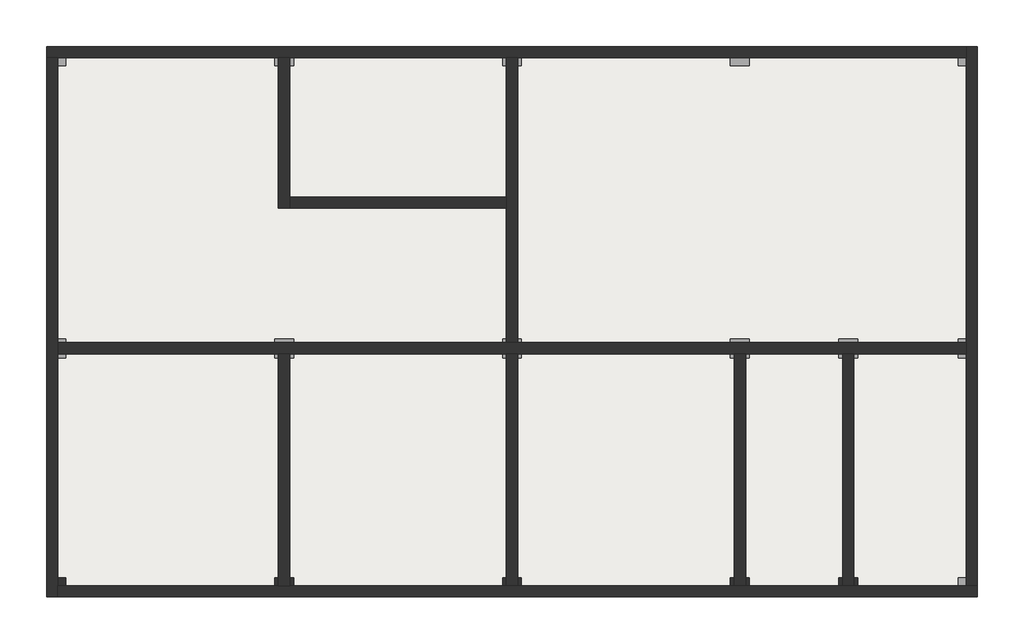
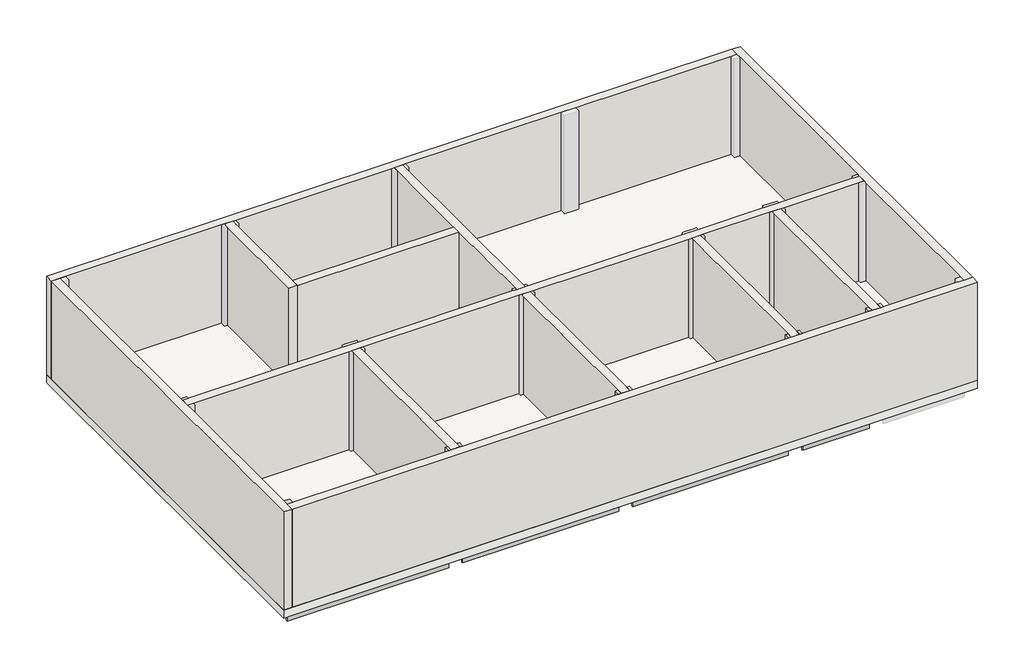
# One storey, part 1 of 2: 12 walls, 8 beams, 5 columns, 1 slab.
"""IFC4 building model written with IfcOpenShell, lengths in millimetres."""

import ifcopenshell
import ifcopenshell.guid

model = None  # the IFC model being written
_history = None  # IfcOwnerHistory: only IFC2X3 demands one
_inside = {}  # id of a spatial element -> (the spatial element, [elements in it])
_under = {}  # id of a project, library or spatial element -> (it, [spatial elements below it])
_declared = {}  # id of a project -> (the project, [libraries it declares])
_typed = {}  # id of a type object -> (the type object, [elements of that type])
_made_of = {}  # id of a material, layer set ... -> (it, [elements and type objects made of it])


def new_model(schema):
    """Start an empty IFC model of exactly this schema.

    Asked for "IFC4X3", IfcOpenShell would pick the latest addendum, in which some entities
    have other attributes; the version numbers below select the first issue.
    IFC2X3 requires an IfcOwnerHistory on every rooted entity: one is made here for all.
    """
    global model, _history
    if schema == "IFC4X3":
        model = ifcopenshell.file(schema_version=(4, 3, 0, 0))
    else:
        model = ifcopenshell.file(schema=schema)
    _inside.clear()
    _under.clear()
    _declared.clear()
    _typed.clear()
    _made_of.clear()
    _history = None
    if model.schema == "IFC2X3":
        org = make("IfcOrganization", Name="unknown")
        user = make(
            "IfcPersonAndOrganization",
            ThePerson=make("IfcPerson", FamilyName="unknown"),
            TheOrganization=org,
        )
        app = make(
            "IfcApplication",
            ApplicationDeveloper=org,
            Version="unknown",
            ApplicationFullName="unknown",
            ApplicationIdentifier="unknown",
        )
        _history = make(
            "IfcOwnerHistory",
            OwningUser=user,
            OwningApplication=app,
            ChangeAction="ADDED",
            CreationDate=0,
        )
    return model


def make(cls, **values):
    """One entity of the class cls with the attributes given. An attribute that is None is left unset."""
    return model.create_entity(
        cls, **{name: value for name, value in values.items() if value is not None}
    )


def rooted(cls, **values):
    """An entity with a GlobalId (a new one), such as an element, a storey or a relation."""
    return make(cls, GlobalId=ifcopenshell.guid.new(), OwnerHistory=_history, **values)


def si_unit(unit_type, name, prefix=None):
    """IfcSIUnit, for example si_unit("LENGTHUNIT", "METRE", prefix="MILLI")."""
    return make("IfcSIUnit", UnitType=unit_type, Prefix=prefix, Name=name)


def assignment(units):
    """IfcUnitAssignment: the units of a project."""
    return None if units is None else make("IfcUnitAssignment", Units=units)


def point(xyz):
    """IfcCartesianPoint."""
    return None if xyz is None else make("IfcCartesianPoint", Coordinates=xyz)


def direction(xyz):
    """IfcDirection."""
    return None if xyz is None else make("IfcDirection", DirectionRatios=xyz)


def frame(location, z_axis=None, x_axis=None):
    """IfcAxis2Placement3D, a coordinate frame: its origin and axes. An axis left out is left unset."""
    return make(
        "IfcAxis2Placement3D",
        Location=point(location),
        Axis=direction(z_axis),
        RefDirection=direction(x_axis),
    )


def origin():
    """The frame at (0, 0, 0) with its axes left unset."""
    return frame((0.0, 0.0, 0.0))


def place(relative_to, where):
    """IfcLocalPlacement: puts the frame where relative to a parent placement (None: the world)."""
    return make(
        "IfcLocalPlacement", PlacementRelTo=relative_to, RelativePlacement=where
    )


def context(
    kind, dimensions, precision=None, world=None, true_north=None, identifier=None
):
    """IfcGeometricRepresentationContext, for example the 3D "Model" context."""
    return make(
        "IfcGeometricRepresentationContext",
        ContextIdentifier=identifier,
        ContextType=kind,
        CoordinateSpaceDimension=dimensions,
        Precision=precision,
        WorldCoordinateSystem=world,
        TrueNorth=true_north,
    )


def project(units=None, contexts=None):
    """IfcProject with its units and contexts."""
    return rooted(
        "IfcProject",
        Name="project",
        RepresentationContexts=contexts,
        UnitsInContext=assignment(units),
    )


def spatial(cls, under=None, at=None, **own):
    """A site, building, storey or space (cls), placed at a placement, below another one or the project."""
    s = rooted(cls, ObjectPlacement=at, **own)
    if under is not None:
        _under.setdefault(under.id(), (under, []))[1].append(s)
    return s


def polyline(points):
    """IfcPolyline through the points."""
    return make("IfcPolyline", Points=[point(p) for p in points])


def outline(outer, holes=None, kind="AREA"):
    """IfcArbitraryClosedProfileDef: a profile drawn as a closed curve; with holes, ...WithVoids."""
    if holes is None:
        return make("IfcArbitraryClosedProfileDef", ProfileType=kind, OuterCurve=outer)
    return make(
        "IfcArbitraryProfileDefWithVoids",
        ProfileType=kind,
        OuterCurve=outer,
        InnerCurves=holes,
    )


def extrude(swept, where, along, depth):
    """IfcExtrudedAreaSolid: the profile swept, set in the frame where, extruded along a direction by depth."""
    return make(
        "IfcExtrudedAreaSolid",
        SweptArea=swept,
        Position=where,
        ExtrudedDirection=direction(along),
        Depth=depth,
    )


def faces_of(points, faces, orient=None, outer=None):
    """IfcFace entities. A face is a list of loops; a loop is a list of indices into points, from 0.

    orient and outer hold one flag for each loop. By default every Orientation is true, the
    first loop of a face is its IfcFaceOuterBound and the others are IfcFaceBound.
    """
    made = []
    for i, loops in enumerate(faces):
        bounds = []
        for j, loop in enumerate(loops):
            is_outer = j == 0 if outer is None else outer[i][j]
            bounds.append(
                make(
                    "IfcFaceOuterBound" if is_outer else "IfcFaceBound",
                    Bound=make("IfcPolyLoop", Polygon=[points[k] for k in loop]),
                    Orientation=True if orient is None else orient[i][j],
                )
            )
        made.append(make("IfcFace", Bounds=bounds))
    return made


def faceted_brep(points, faces, orient=None, outer=None, voids=None):
    """IfcFacetedBrep: a solid bounded by flat faces; with voids (closed shells), ...WithVoids."""
    shared = [point(p) for p in points]
    hull = make("IfcClosedShell", CfsFaces=faces_of(shared, faces, orient, outer))
    if voids is None:
        return make("IfcFacetedBrep", Outer=hull)
    return make(
        "IfcFacetedBrepWithVoids",
        Outer=hull,
        Voids=[
            make(cls, CfsFaces=faces_of(shared, fs, o, b)) for cls, fs, o, b in voids
        ],
    )


def shape(context_of_items, identifier, shape_type, items):
    """IfcShapeRepresentation: the items that make up one representation, for example the "Body"."""
    return make(
        "IfcShapeRepresentation",
        ContextOfItems=context_of_items,
        RepresentationIdentifier=identifier,
        RepresentationType=shape_type,
        Items=items,
    )


def made_of(thing, what):
    """Note that an element or type object is made of a material, layer set ...; save() writes the relation."""
    if what is not None:
        _made_of.setdefault(what.id(), (what, []))[1].append(thing)
    return thing


def element(
    cls,
    number,
    at=None,
    inside=None,
    cuts=None,
    type_object=None,
    material=None,
    context=None,
    identifier="Body",
    shape_type=None,
    held_by="IfcProductDefinitionShape",
    body=None,
    shapes=None,
    **own,
):
    """One element of the class cls, such as IfcWall. Its Tag is "e" and its number.

    at: its placement. inside: the storey or other place that contains it. cuts: it is an
    opening in that element (IfcRelVoidsElement). A single representation is given by context,
    identifier, shape_type and body (its items); several are given by shapes. held_by: the class
    of the entity that holds the representations. save() writes the other relations.
    """
    e = rooted(cls, Tag="e%d" % number, ObjectPlacement=at, **own)
    if body is not None:
        shapes = [shape(context, identifier, shape_type, body)]
    if shapes is not None:
        e.Representation = make(held_by, Representations=shapes)
    if inside is not None:
        _inside.setdefault(inside.id(), (inside, []))[1].append(e)
    if cuts is not None:
        rooted(
            "IfcRelVoidsElement", RelatingBuildingElement=cuts, RelatedOpeningElement=e
        )
    if type_object is not None:
        _typed.setdefault(type_object.id(), (type_object, []))[1].append(e)
    return made_of(e, material)


def aggregate(whole, parts):
    """IfcRelAggregates: a whole, such as a stair, and the parts it consists of."""
    return rooted("IfcRelAggregates", RelatingObject=whole, RelatedObjects=parts)


def save(model, path):
    """Write the relations noted so far, then the file.

    IfcRelAggregates (storeys below a building ...), IfcRelContainedInSpatialStructure (elements
    in a storey), IfcRelDefinesByType, IfcRelAssociatesMaterial and IfcRelDeclares: one each for
    every whole, place, type object, material and project.
    """
    for whole, parts in _under.values():
        aggregate(whole, parts)
    for where, things in _inside.values():
        rooted(
            "IfcRelContainedInSpatialStructure",
            RelatedElements=things,
            RelatingStructure=where,
        )
    for kind, things in _typed.values():
        rooted("IfcRelDefinesByType", RelatedObjects=things, RelatingType=kind)
    for what, things in _made_of.values():
        rooted("IfcRelAssociatesMaterial", RelatedObjects=things, RelatingMaterial=what)
    for by, libraries in _declared.values():
        rooted("IfcRelDeclares", RelatingContext=by, RelatedDefinitions=libraries)
    model.write(path)


model = new_model("IFC4")

# Units and contexts
model_context = context("Model", 3, world=origin())
ifc_project = project(units=[si_unit("LENGTHUNIT", "METRE", prefix="MILLI")], contexts=[model_context])

# Site, building, storey
site = spatial("IfcSite", under=ifc_project)
building = spatial("IfcBuilding", under=site)
storey = spatial("IfcBuildingStorey", under=building, Name="2nd FL GL+6,200", Elevation=6000.0)

# Beams
placement = place(None, origin())
element("IfcBeam", 1, ObjectType="RC Beam_Rectangular : 350 x 700mm", at=placement, inside=storey, context=model_context, shape_type="SweptSolid", body=[
    extrude(outline(polyline([(-18645.7273237, 1485.9763125), (-18595.7273237, 1485.9763125), (-18595.7273237, -4314.0236875), (-18645.7273237, -4314.0236875), (-18645.7273237, 1485.9763125)])), frame((0.0, 0.0, 5300.0), z_axis=(0.0, 0.0, 1.0), x_axis=(1.0, 0.0, 0.0)), (0.0, 0.0, 1.0), 400.0),
])
element("IfcBeam", 2, ObjectType="RC Beam_Rectangular : 350 x 700mm", at=placement, inside=storey, context=model_context, shape_type="SweptSolid", body=[
    extrude(outline(polyline([(-12545.7273237, 1485.9763125), (-12520.7273237, 1485.9763125), (-12520.7273237, -4314.0236875), (-12545.7273237, -4314.0236875), (-12545.7273237, 1485.9763125)])), frame((0.0, 0.0, 5300.0), z_axis=(0.0, 0.0, 1.0), x_axis=(1.0, 0.0, 0.0)), (0.0, 0.0, 1.0), 400.0),
    extrude(outline(polyline([(-12870.7273237, 1485.9763125), (-12845.7273237, 1485.9763125), (-12845.7273237, -4314.0236875), (-12870.7273237, -4314.0236875), (-12870.7273237, 1485.9763125)])), frame((0.0, 0.0, 5300.0), z_axis=(0.0, 0.0, 1.0), x_axis=(1.0, 0.0, 0.0)), (0.0, 0.0, 1.0), 400.0),
])
element("IfcBeam", 3, ObjectType="RC Beam_Rectangular : 350 x 700mm", at=placement, inside=storey, context=model_context, shape_type="SweptSolid", body=[
    extrude(outline(polyline([(-6545.7273237, 1485.9763125), (-6520.7273237, 1485.9763125), (-6520.7273237, -4314.0236875), (-6545.7273237, -4314.0236875), (-6545.7273237, 1485.9763125)])), frame((0.0, 0.0, 5300.0), z_axis=(0.0, 0.0, 1.0), x_axis=(1.0, 0.0, 0.0)), (0.0, 0.0, 1.0), 400.0),
    extrude(outline(polyline([(-6870.7273237, 1485.9763125), (-6845.7273237, 1485.9763125), (-6845.7273237, -4314.0236875), (-6870.7273237, -4314.0236875), (-6870.7273237, 1485.9763125)])), frame((0.0, 0.0, 5300.0), z_axis=(0.0, 0.0, 1.0), x_axis=(1.0, 0.0, 0.0)), (0.0, 0.0, 1.0), 400.0),
])
element("IfcBeam", 4, ObjectType="RC Beam_Rectangular : 350 x 700mm", at=placement, inside=storey, context=model_context, shape_type="SweptSolid", body=[
    extrude(outline(polyline([(-545.7273237, 1485.9763125), (-520.7273237, 1485.9763125), (-520.7273237, -4314.0236875), (-545.7273237, -4314.0236875), (-545.7273237, 1485.9763125)])), frame((0.0, 0.0, 5300.0), z_axis=(0.0, 0.0, 1.0), x_axis=(1.0, 0.0, 0.0)), (0.0, 0.0, 1.0), 400.0),
    extrude(outline(polyline([(-870.7273237, 1485.9763125), (-845.7273237, 1485.9763125), (-845.7273237, -4314.0236875), (-870.7273237, -4314.0236875), (-870.7273237, 1485.9763125)])), frame((0.0, 0.0, 5300.0), z_axis=(0.0, 0.0, 1.0), x_axis=(1.0, 0.0, 0.0)), (0.0, 0.0, 1.0), 400.0),
])
element("IfcBeam", 5, ObjectType="RC Beam_Rectangular : 350 x 700mm", at=placement, inside=storey, context=model_context, shape_type="SweptSolid", body=[
    extrude(outline(polyline([(-12945.7273237, -4514.0236875), (-18645.7273237, -4514.0236875), (-18645.7273237, -4464.0236875), (-12945.7273237, -4464.0236875), (-12945.7273237, -4514.0236875)])), frame((0.0, 0.0, 5300.0), z_axis=(0.0, 0.0, 1.0), x_axis=(1.0, 0.0, 0.0)), (0.0, 0.0, 1.0), 400.0),
])
element("IfcBeam", 6, ObjectType="RC Beam_Rectangular : 350 x 700mm", at=placement, inside=storey, context=model_context, shape_type="SweptSolid", body=[
    extrude(outline(polyline([(-12445.7273237, -4514.0236875), (-12445.7273237, -4464.0236875), (-6945.7273237, -4464.0236875), (-6945.7273237, -4514.0236875), (-12445.7273237, -4514.0236875)])), frame((0.0, 0.0, 5300.0), z_axis=(0.0, 0.0, 1.0), x_axis=(1.0, 0.0, 0.0)), (0.0, 0.0, 1.0), 400.0),
])
element("IfcBeam", 7, ObjectType="RC Beam_Rectangular : 350 x 700mm", at=placement, inside=storey, context=model_context, shape_type="SweptSolid", body=[
    extrude(outline(polyline([(-6445.7273237, -4514.0236875), (-6445.7273237, -4464.0236875), (-945.7273237, -4464.0236875), (-945.7273237, -4514.0236875), (-6445.7273237, -4514.0236875)])), frame((0.0, 0.0, 5300.0), z_axis=(0.0, 0.0, 1.0), x_axis=(1.0, 0.0, 0.0)), (0.0, 0.0, 1.0), 400.0),
])
element("IfcBeam", 8, ObjectType="RC Beam_Rectangular : 350 x 700mm", at=placement, inside=storey, context=model_context, shape_type="SweptSolid", body=[
    extrude(outline(polyline([(-445.7273237, -4514.0236875), (-445.7273237, -4464.0236875), (1904.2726763, -4464.0236875), (1904.2726763, -4514.0236875), (-445.7273237, -4514.0236875)])), frame((0.0, 0.0, 5300.0), z_axis=(0.0, 0.0, 1.0), x_axis=(1.0, 0.0, 0.0)), (0.0, 0.0, 1.0), 400.0),
])

# Columns
element("IfcColumn", 9, ObjectType="RC_Column_Rectangular : 500 x 500mm", at=placement, inside=storey, context=model_context, shape_type="Brep", body=[
    faceted_brep([(-18645.7273237, -4314.0236875, 6000.0), (-18445.7273237, -4314.0236875, 6000.0), (-18445.7273237, -4514.0236875, 6000.0), (-18645.7273237, -4514.0236875, 6000.0), (-18445.7273237, -4314.0236875, 9667.0), (-18645.7273237, -4314.0236875, 9300.0), (-18645.7273237, -4314.0236875, 9667.0), (-18595.7273237, -4314.0236875, 9667.0), (-18445.7273237, -4514.0236875, 9667.0), (-18645.7273237, -4514.0236875, 9667.0)], [[[0, 1, 2, 3]], [[4, 1, 0, 5, 6, 7]], [[1, 4, 8, 2]], [[4, 7, 6, 9, 8]], [[6, 5, 0, 3, 9]], [[3, 2, 8, 9]]]),
])
element("IfcColumn", 10, ObjectType="RC_Column_Rectangular : 500 x 500mm", at=placement, inside=storey, context=model_context, shape_type="Brep", body=[
    faceted_brep([(-12945.7273237, -4514.0236875, 6000.0), (-12945.7273237, -4314.0236875, 6000.0), (-12845.7273237, -4314.0236875, 6000.0), (-12845.7273237, -4514.0236875, 6000.0), (-12945.7273237, -4314.0236875, 9667.0), (-12945.7273237, -4514.0236875, 9300.0), (-12945.7273237, -4514.0236875, 9667.0), (-12945.7273237, -4464.0236875, 9667.0), (-12845.7273237, -4514.0236875, 9667.0), (-12845.7273237, -4314.0236875, 9667.0), (-12870.7273237, -4314.0236875, 9667.0), (-12845.7273237, -4314.0236875, 9300.0)], [[[0, 1, 2, 3]], [[4, 1, 0, 5, 6, 7]], [[4, 7, 6, 8, 9, 10]], [[3, 2, 11, 9, 8]], [[1, 4, 10, 9, 11, 2]], [[6, 5, 0, 3, 8]]]),
    faceted_brep([(-12445.7273237, -4314.0236875, 9667.0), (-12445.7273237, -4314.0236875, 6000.0), (-12545.7273237, -4314.0236875, 6000.0), (-12545.7273237, -4314.0236875, 9300.0), (-12545.7273237, -4314.0236875, 9667.0), (-12520.7273237, -4314.0236875, 9667.0), (-12445.7273237, -4464.0236875, 9667.0), (-12445.7273237, -4514.0236875, 9667.0), (-12445.7273237, -4514.0236875, 9300.0), (-12445.7273237, -4514.0236875, 6000.0), (-12545.7273237, -4514.0236875, 9667.0), (-12545.7273237, -4514.0236875, 6000.0)], [[[0, 1, 2, 3, 4, 5]], [[1, 0, 6, 7, 8, 9]], [[9, 8, 7, 10, 11]], [[2, 11, 10, 4, 3]], [[1, 9, 11, 2]], [[7, 6, 0, 5, 4, 10]]]),
])
element("IfcColumn", 11, ObjectType="RC_Column_Rectangular : 500 x 500mm", at=placement, inside=storey, context=model_context, shape_type="Brep", body=[
    faceted_brep([(-6945.7273237, -4514.0236875, 6000.0), (-6945.7273237, -4314.0236875, 6000.0), (-6845.7273237, -4314.0236875, 6000.0), (-6845.7273237, -4514.0236875, 6000.0), (-6945.7273237, -4314.0236875, 9667.0), (-6945.7273237, -4514.0236875, 9300.0), (-6945.7273237, -4514.0236875, 9667.0), (-6945.7273237, -4464.0236875, 9667.0), (-6845.7273237, -4514.0236875, 9667.0), (-6845.7273237, -4314.0236875, 9667.0), (-6870.7273237, -4314.0236875, 9667.0), (-6845.7273237, -4314.0236875, 9300.0)], [[[0, 1, 2, 3]], [[4, 1, 0, 5, 6, 7]], [[4, 7, 6, 8, 9, 10]], [[3, 2, 11, 9, 8]], [[1, 4, 10, 9, 11, 2]], [[6, 5, 0, 3, 8]]]),
    faceted_brep([(-6445.7273237, -4314.0236875, 9667.0), (-6445.7273237, -4314.0236875, 6000.0), (-6545.7273237, -4314.0236875, 6000.0), (-6545.7273237, -4314.0236875, 9300.0), (-6545.7273237, -4314.0236875, 9667.0), (-6520.7273237, -4314.0236875, 9667.0), (-6445.7273237, -4464.0236875, 9667.0), (-6445.7273237, -4514.0236875, 9667.0), (-6445.7273237, -4514.0236875, 9300.0), (-6445.7273237, -4514.0236875, 6000.0), (-6545.7273237, -4514.0236875, 9667.0), (-6545.7273237, -4514.0236875, 6000.0)], [[[0, 1, 2, 3, 4, 5]], [[1, 0, 6, 7, 8, 9]], [[9, 8, 7, 10, 11]], [[2, 11, 10, 4, 3]], [[1, 9, 11, 2]], [[7, 6, 0, 5, 4, 10]]]),
])
element("IfcColumn", 12, ObjectType="RC_Column_Rectangular : 500 x 500mm", at=placement, inside=storey, context=model_context, shape_type="Brep", body=[
    faceted_brep([(-945.7273237, -4514.0236875, 6000.0), (-945.7273237, -4314.0236875, 6000.0), (-845.7273237, -4314.0236875, 6000.0), (-845.7273237, -4514.0236875, 6000.0), (-945.7273237, -4314.0236875, 9667.0), (-945.7273237, -4514.0236875, 9300.0), (-945.7273237, -4514.0236875, 9667.0), (-945.7273237, -4464.0236875, 9667.0), (-845.7273237, -4514.0236875, 9667.0), (-845.7273237, -4314.0236875, 9667.0), (-870.7273237, -4314.0236875, 9667.0), (-845.7273237, -4314.0236875, 9300.0)], [[[0, 1, 2, 3]], [[4, 1, 0, 5, 6, 7]], [[4, 7, 6, 8, 9, 10]], [[3, 2, 11, 9, 8]], [[1, 4, 10, 9, 11, 2]], [[6, 5, 0, 3, 8]]]),
    faceted_brep([(-445.7273237, -4314.0236875, 9667.0), (-445.7273237, -4314.0236875, 6000.0), (-545.7273237, -4314.0236875, 6000.0), (-545.7273237, -4314.0236875, 9300.0), (-545.7273237, -4314.0236875, 9667.0), (-520.7273237, -4314.0236875, 9667.0), (-445.7273237, -4464.0236875, 9667.0), (-445.7273237, -4514.0236875, 9667.0), (-445.7273237, -4514.0236875, 9300.0), (-445.7273237, -4514.0236875, 6000.0), (-545.7273237, -4514.0236875, 9667.0), (-545.7273237, -4514.0236875, 6000.0)], [[[0, 1, 2, 3, 4, 5]], [[1, 0, 6, 7, 8, 9]], [[9, 8, 7, 10, 11]], [[2, 11, 10, 4, 3]], [[1, 9, 11, 2]], [[7, 6, 0, 5, 4, 10]]]),
])
element("IfcColumn", 13, ObjectType="RC_Column_Rectangular : 500 x 500mm", at=placement, inside=storey, context=model_context, shape_type="Brep", body=[
    faceted_brep([(1904.2726763, -4514.0236875, 6000.0), (1904.2726763, -4314.0236875, 6000.0), (2004.2726763, -4314.0236875, 6000.0), (2004.2726763, -4514.0236875, 6000.0), (1904.2726763, -4314.0236875, 9667.0), (1904.2726763, -4514.0236875, 9300.0), (1904.2726763, -4514.0236875, 9667.0), (1904.2726763, -4464.0236875, 9667.0), (2004.2726763, -4514.0236875, 9667.0), (2004.2726763, -4314.0236875, 9667.0), (1979.2726763, -4314.0236875, 9667.0), (2004.2726763, -4314.0236875, 9300.0)], [[[0, 1, 2, 3]], [[4, 1, 0, 5, 6, 7]], [[4, 7, 6, 8, 9, 10]], [[3, 2, 11, 9, 8]], [[1, 4, 10, 9, 11, 2]], [[6, 5, 0, 3, 8]]]),
    faceted_brep([(2404.2726763, -4314.0236875, 9667.0), (2404.2726763, -4314.0236875, 6000.0), (2304.2726763, -4314.0236875, 6000.0), (2304.2726763, -4314.0236875, 9300.0), (2304.2726763, -4314.0236875, 9667.0), (2329.2726763, -4314.0236875, 9667.0), (2404.2726763, -4464.0236875, 9667.0), (2404.2726763, -4514.0236875, 9667.0), (2404.2726763, -4514.0236875, 9300.0), (2404.2726763, -4514.0236875, 6000.0), (2304.2726763, -4514.0236875, 9667.0), (2304.2726763, -4514.0236875, 6000.0)], [[[0, 1, 2, 3, 4, 5]], [[1, 0, 6, 7, 8, 9]], [[9, 8, 7, 10, 11]], [[2, 11, 10, 4, 3]], [[1, 9, 11, 2]], [[7, 6, 0, 5, 4, 10]]]),
])

# Slab
element("IfcSlab", 14, ObjectType="H_FL_ACS_RC Slab_T150", at=placement, inside=storey, context=model_context, shape_type="Brep", body=[
    faceted_brep([(5554.2726763, -4814.0236875, 5700.0), (-18645.7273237, -4814.0236875, 5700.0), (-18945.7273237, -4814.0236875, 5700.0), (-18945.7273237, 9385.9763125, 5700.0), (-18945.7273237, 9685.9763125, 5700.0), (5254.2726763, 9685.9763125, 5700.0), (5554.2726763, 9685.9763125, 5700.0), (5554.2726763, -4514.0236875, 5700.0), (5554.2726763, -4814.0236875, 6000.0), (5554.2726763, 9685.9763125, 6000.0), (-18945.7273237, 9685.9763125, 6000.0), (-18945.7273237, -4814.0236875, 6000.0)], [[[0, 1, 2, 3, 4, 5, 6, 7]], [[8, 9, 10, 11]], [[2, 1, 0, 8, 11]], [[4, 3, 2, 11, 10]], [[6, 5, 4, 10, 9]], [[0, 7, 6, 9, 8]]]),
])

# Walls
element("IfcWall", 15, ObjectType="일반 - 300mm", at=placement, inside=storey, context=model_context, shape_type="Brep", body=[
    faceted_brep([(-18945.7273237, 9385.9763125, 6000.0), (-18645.7273237, 9385.9763125, 6000.0), (-18445.7273237, 9385.9763125, 6000.0), (-12945.7273237, 9385.9763125, 6000.0), (-12845.7273237, 9385.9763125, 6000.0), (-12545.7273237, 9385.9763125, 6000.0), (-12445.7273237, 9385.9763125, 6000.0), (-6945.7273237, 9385.9763125, 6000.0), (-6845.7273237, 9385.9763125, 6000.0), (-6545.7273237, 9385.9763125, 6000.0), (-6445.7273237, 9385.9763125, 6000.0), (-945.7273237, 9385.9763125, 6000.0), (-445.7273237, 9385.9763125, 6000.0), (5054.2726763, 9385.9763125, 6000.0), (5254.2726763, 9385.9763125, 6000.0), (5254.2726763, 9385.9763125, 9300.0), (5254.2726763, 9385.9763125, 9667.0), (5054.2726763, 9385.9763125, 9667.0), (-445.7273237, 9385.9763125, 9667.0), (-945.7273237, 9385.9763125, 9667.0), (-6445.7273237, 9385.9763125, 9667.0), (-6545.7273237, 9385.9763125, 9667.0), (-6845.7273237, 9385.9763125, 9667.0), (-6945.7273237, 9385.9763125, 9667.0), (-12445.7273237, 9385.9763125, 9667.0), (-12545.7273237, 9385.9763125, 9667.0), (-12845.7273237, 9385.9763125, 9667.0), (-12945.7273237, 9385.9763125, 9667.0), (-18445.7273237, 9385.9763125, 9667.0), (-18645.7273237, 9385.9763125, 9667.0), (-18945.7273237, 9385.9763125, 9667.0), (5254.2726763, 9685.9763125, 6000.0), (-18945.7273237, 9685.9763125, 6000.0), (-18945.7273237, 9685.9763125, 9667.0), (5254.2726763, 9685.9763125, 9667.0)], [[[0, 1, 2, 3, 4, 5, 6, 7, 8, 9, 10, 11, 12, 13, 14, 15, 16, 17, 18, 19, 20, 21, 22, 23, 24, 25, 26, 27, 28, 29, 30]], [[31, 32, 33, 34]], [[14, 13, 12, 11, 10, 9, 8, 7, 6, 5, 4, 3, 2, 1, 0, 32, 31]], [[32, 0, 30, 33]], [[14, 31, 34, 16, 15]], [[30, 29, 28, 27, 26, 25, 24, 23, 22, 21, 20, 19, 18, 17, 16, 34, 33]]]),
])
element("IfcWall", 16, ObjectType="일반 - 300mm", at=placement, inside=storey, context=model_context, shape_type="Brep", body=[
    faceted_brep([(-18645.7273237, -4814.0236875, 6000.0), (-18645.7273237, -4514.0236875, 6000.0), (-18645.7273237, -4314.0236875, 6000.0), (-18645.7273237, 1485.9763125, 6000.0), (-18645.7273237, 1585.9763125, 6000.0), (-18645.7273237, 1885.9763125, 6000.0), (-18645.7273237, 1985.9763125, 6000.0), (-18645.7273237, 9185.9763125, 6000.0), (-18645.7273237, 9385.9763125, 6000.0), (-18645.7273237, 9385.9763125, 9667.0), (-18645.7273237, 9185.9763125, 9667.0), (-18645.7273237, 1985.9763125, 9667.0), (-18645.7273237, 1885.9763125, 9667.0), (-18645.7273237, 1585.9763125, 9667.0), (-18645.7273237, 1485.9763125, 9667.0), (-18645.7273237, -4314.0236875, 9667.0), (-18645.7273237, -4514.0236875, 9667.0), (-18645.7273237, -4814.0236875, 9667.0), (-18945.7273237, 9385.9763125, 6000.0), (-18945.7273237, -4814.0236875, 6000.0), (-18945.7273237, -4814.0236875, 9667.0), (-18945.7273237, 9385.9763125, 9667.0)], [[[0, 1, 2, 3, 4, 5, 6, 7, 8, 9, 10, 11, 12, 13, 14, 15, 16, 17]], [[18, 19, 20, 21]], [[8, 7, 6, 5, 4, 3, 2, 1, 0, 19, 18]], [[19, 0, 17, 20]], [[8, 18, 21, 9]], [[17, 16, 15, 14, 13, 12, 11, 10, 9, 21, 20]]]),
])
element("IfcWall", 17, ObjectType="일반 - 300mm", at=placement, inside=storey, context=model_context, shape_type="Brep", body=[
    faceted_brep([(5554.2726763, -4514.0236875, 6000.0), (5254.2726763, -4514.0236875, 6000.0), (5054.2726763, -4514.0236875, 6000.0), (2404.2726763, -4514.0236875, 6000.0), (2304.2726763, -4514.0236875, 6000.0), (2004.2726763, -4514.0236875, 6000.0), (1904.2726763, -4514.0236875, 6000.0), (-445.7273237, -4514.0236875, 6000.0), (-545.7273237, -4514.0236875, 6000.0), (-845.7273237, -4514.0236875, 6000.0), (-945.7273237, -4514.0236875, 6000.0), (-6445.7273237, -4514.0236875, 6000.0), (-6545.7273237, -4514.0236875, 6000.0), (-6845.7273237, -4514.0236875, 6000.0), (-6945.7273237, -4514.0236875, 6000.0), (-12445.7273237, -4514.0236875, 6000.0), (-12545.7273237, -4514.0236875, 6000.0), (-12845.7273237, -4514.0236875, 6000.0), (-12945.7273237, -4514.0236875, 6000.0), (-18445.7273237, -4514.0236875, 6000.0), (-18645.7273237, -4514.0236875, 6000.0), (-18645.7273237, -4514.0236875, 9300.0), (-18645.7273237, -4514.0236875, 9667.0), (-18445.7273237, -4514.0236875, 9667.0), (-12945.7273237, -4514.0236875, 9667.0), (-12845.7273237, -4514.0236875, 9667.0), (-12545.7273237, -4514.0236875, 9667.0), (-12445.7273237, -4514.0236875, 9667.0), (-6945.7273237, -4514.0236875, 9667.0), (-6845.7273237, -4514.0236875, 9667.0), (-6545.7273237, -4514.0236875, 9667.0), (-6445.7273237, -4514.0236875, 9667.0), (-945.7273237, -4514.0236875, 9667.0), (-845.7273237, -4514.0236875, 9667.0), (-545.7273237, -4514.0236875, 9667.0), (-445.7273237, -4514.0236875, 9667.0), (1904.2726763, -4514.0236875, 9667.0), (2004.2726763, -4514.0236875, 9667.0), (2304.2726763, -4514.0236875, 9667.0), (2404.2726763, -4514.0236875, 9667.0), (5054.2726763, -4514.0236875, 9667.0), (5254.2726763, -4514.0236875, 9667.0), (5554.2726763, -4514.0236875, 9667.0), (-18645.7273237, -4814.0236875, 6000.0), (5554.2726763, -4814.0236875, 6000.0), (5554.2726763, -4814.0236875, 9667.0), (-18645.7273237, -4814.0236875, 9667.0)], [[[0, 1, 2, 3, 4, 5, 6, 7, 8, 9, 10, 11, 12, 13, 14, 15, 16, 17, 18, 19, 20, 21, 22, 23, 24, 25, 26, 27, 28, 29, 30, 31, 32, 33, 34, 35, 36, 37, 38, 39, 40, 41, 42]], [[43, 44, 45, 46]], [[20, 19, 18, 17, 16, 15, 14, 13, 12, 11, 10, 9, 8, 7, 6, 5, 4, 3, 2, 1, 0, 44, 43]], [[44, 0, 42, 45]], [[20, 43, 46, 22, 21]], [[42, 41, 40, 39, 38, 37, 36, 35, 34, 33, 32, 31, 30, 29, 28, 27, 26, 25, 24, 23, 22, 46, 45]]]),
])
element("IfcWall", 18, ObjectType="일반 - 300mm", at=placement, inside=storey, context=model_context, shape_type="Brep", body=[
    faceted_brep([(5254.2726763, 9685.9763125, 6000.0), (5254.2726763, 9385.9763125, 6000.0), (5254.2726763, 9185.9763125, 6000.0), (5254.2726763, 1985.9763125, 6000.0), (5254.2726763, 1885.9763125, 6000.0), (5254.2726763, 1585.9763125, 6000.0), (5254.2726763, 1485.9763125, 6000.0), (5254.2726763, -4314.0236875, 6000.0), (5254.2726763, -4514.0236875, 6000.0), (5254.2726763, -4514.0236875, 9667.0), (5254.2726763, -4314.0236875, 9667.0), (5254.2726763, 1485.9763125, 9667.0), (5254.2726763, 1585.9763125, 9667.0), (5254.2726763, 1885.9763125, 9667.0), (5254.2726763, 1985.9763125, 9667.0), (5254.2726763, 9185.9763125, 9667.0), (5254.2726763, 9385.9763125, 9667.0), (5254.2726763, 9685.9763125, 9667.0), (5554.2726763, -4514.0236875, 6000.0), (5554.2726763, 9685.9763125, 6000.0), (5554.2726763, 9685.9763125, 9667.0), (5554.2726763, -4514.0236875, 9667.0)], [[[0, 1, 2, 3, 4, 5, 6, 7, 8, 9, 10, 11, 12, 13, 14, 15, 16, 17]], [[18, 19, 20, 21]], [[8, 7, 6, 5, 4, 3, 2, 1, 0, 19, 18]], [[19, 0, 17, 20]], [[8, 18, 21, 9]], [[17, 16, 15, 14, 13, 12, 11, 10, 9, 21, 20]]]),
])
element("IfcWall", 19, ObjectType="일반 - 300mm", at=placement, inside=storey, context=model_context, shape_type="Brep", body=[
    faceted_brep([(-12545.7273237, 5425.9613486, 6000.0), (-12545.7273237, 5725.9613486, 6000.0), (-12545.7273237, 9185.9763125, 6000.0), (-12545.7273237, 9385.9763125, 6000.0), (-12545.7273237, 9385.9763125, 9667.0), (-12545.7273237, 9185.9763125, 9667.0), (-12545.7273237, 5725.9613486, 9667.0), (-12545.7273237, 5425.9613486, 9667.0), (-12845.7273237, 9385.9763125, 6000.0), (-12845.7273237, 9185.9763125, 6000.0), (-12845.7273237, 5425.9613486, 6000.0), (-12845.7273237, 5425.9613486, 9300.0), (-12845.7273237, 5425.9613486, 9667.0), (-12845.7273237, 9185.9763125, 9667.0), (-12845.7273237, 9385.9763125, 9667.0)], [[[0, 1, 2, 3, 4, 5, 6, 7]], [[8, 9, 10, 11, 12, 13, 14]], [[3, 2, 1, 0, 10, 9, 8]], [[3, 8, 14, 4]], [[10, 0, 7, 12, 11]], [[7, 6, 5, 4, 14, 13, 12]]]),
])
element("IfcWall", 20, ObjectType="일반 - 300mm", at=placement, inside=storey, context=model_context, shape_type="Brep", body=[
    faceted_brep([(-12545.7273237, 5425.9613486, 6000.0), (-6845.7273237, 5425.9613486, 6000.0), (-6845.7273237, 5425.9613486, 9300.0), (-6845.7273237, 5425.9613486, 9667.0), (-6870.7273237, 5425.9613486, 9667.0), (-12520.7273237, 5425.9613486, 9667.0), (-12545.7273237, 5425.9613486, 9667.0), (-6845.7273237, 5725.9613486, 6000.0), (-12545.7273237, 5725.9613486, 6000.0), (-12545.7273237, 5725.9613486, 9300.0), (-12545.7273237, 5725.9613486, 9667.0), (-12520.7273237, 5725.9613486, 9667.0), (-6870.7273237, 5725.9613486, 9667.0), (-6845.7273237, 5725.9613486, 9667.0), (-6845.7273237, 5725.9613486, 9300.0)], [[[0, 1, 2, 3, 4, 5, 6]], [[7, 8, 9, 10, 11, 12, 13, 14]], [[1, 0, 8, 7]], [[8, 0, 6, 10, 9]], [[1, 7, 14, 13, 3, 2]], [[6, 5, 4, 3, 13, 12, 11, 10]]]),
])
element("IfcWall", 21, ObjectType="일반 - 300mm", at=placement, inside=storey, context=model_context, shape_type="Brep", body=[
    faceted_brep([(-6545.7273237, 1885.9763125, 6000.0), (-6545.7273237, 1985.9763125, 6000.0), (-6545.7273237, 9185.9763125, 6000.0), (-6545.7273237, 9385.9763125, 6000.0), (-6545.7273237, 9385.9763125, 9667.0), (-6545.7273237, 9185.9763125, 9667.0), (-6545.7273237, 1985.9763125, 9667.0), (-6545.7273237, 1885.9763125, 9667.0), (-6845.7273237, 9385.9763125, 6000.0), (-6845.7273237, 9185.9763125, 6000.0), (-6845.7273237, 5725.9613486, 6000.0), (-6845.7273237, 5425.9613486, 6000.0), (-6845.7273237, 1985.9763125, 6000.0), (-6845.7273237, 1885.9763125, 6000.0), (-6845.7273237, 1885.9763125, 9667.0), (-6845.7273237, 1985.9763125, 9667.0), (-6845.7273237, 5425.9613486, 9667.0), (-6845.7273237, 5725.9613486, 9667.0), (-6845.7273237, 9185.9763125, 9667.0), (-6845.7273237, 9385.9763125, 9667.0)], [[[0, 1, 2, 3, 4, 5, 6, 7]], [[8, 9, 10, 11, 12, 13, 14, 15, 16, 17, 18, 19]], [[3, 2, 1, 0, 13, 12, 11, 10, 9, 8]], [[3, 8, 19, 4]], [[13, 0, 7, 14]], [[7, 6, 5, 4, 19, 18, 17, 16, 15, 14]]]),
])
element("IfcWall", 22, ObjectType="일반 - 300mm", at=placement, inside=storey, context=model_context, shape_type="Brep", body=[
    faceted_brep([(-18645.7273237, 1585.9763125, 6000.0), (-18445.7273237, 1585.9763125, 6000.0), (-12945.7273237, 1585.9763125, 6000.0), (-12845.7273237, 1585.9763125, 6000.0), (-12545.7273237, 1585.9763125, 6000.0), (-12445.7273237, 1585.9763125, 6000.0), (-6945.7273237, 1585.9763125, 6000.0), (-6845.7273237, 1585.9763125, 6000.0), (-6545.7273237, 1585.9763125, 6000.0), (-6445.7273237, 1585.9763125, 6000.0), (-945.7273237, 1585.9763125, 6000.0), (-845.7273237, 1585.9763125, 6000.0), (-545.7273237, 1585.9763125, 6000.0), (-445.7273237, 1585.9763125, 6000.0), (1904.2726763, 1585.9763125, 6000.0), (2004.2726763, 1585.9763125, 6000.0), (2304.2726763, 1585.9763125, 6000.0), (2404.2726763, 1585.9763125, 6000.0), (5054.2726763, 1585.9763125, 6000.0), (5254.2726763, 1585.9763125, 6000.0), (5254.2726763, 1585.9763125, 9667.0), (5054.2726763, 1585.9763125, 9667.0), (2404.2726763, 1585.9763125, 9667.0), (2304.2726763, 1585.9763125, 9667.0), (2004.2726763, 1585.9763125, 9667.0), (1904.2726763, 1585.9763125, 9667.0), (-445.7273237, 1585.9763125, 9667.0), (-545.7273237, 1585.9763125, 9667.0), (-845.7273237, 1585.9763125, 9667.0), (-945.7273237, 1585.9763125, 9667.0), (-6445.7273237, 1585.9763125, 9667.0), (-6545.7273237, 1585.9763125, 9667.0), (-6845.7273237, 1585.9763125, 9667.0), (-6945.7273237, 1585.9763125, 9667.0), (-12445.7273237, 1585.9763125, 9667.0), (-12545.7273237, 1585.9763125, 9667.0), (-12845.7273237, 1585.9763125, 9667.0), (-12945.7273237, 1585.9763125, 9667.0), (-18445.7273237, 1585.9763125, 9667.0), (-18645.7273237, 1585.9763125, 9667.0), (5254.2726763, 1885.9763125, 6000.0), (5054.2726763, 1885.9763125, 6000.0), (2404.2726763, 1885.9763125, 6000.0), (1904.2726763, 1885.9763125, 6000.0), (-445.7273237, 1885.9763125, 6000.0), (-945.7273237, 1885.9763125, 6000.0), (-6445.7273237, 1885.9763125, 6000.0), (-6545.7273237, 1885.9763125, 6000.0), (-6845.7273237, 1885.9763125, 6000.0), (-6945.7273237, 1885.9763125, 6000.0), (-12445.7273237, 1885.9763125, 6000.0), (-12945.7273237, 1885.9763125, 6000.0), (-18445.7273237, 1885.9763125, 6000.0), (-18645.7273237, 1885.9763125, 6000.0), (-18645.7273237, 1885.9763125, 9667.0), (-18445.7273237, 1885.9763125, 9667.0), (-12945.7273237, 1885.9763125, 9667.0), (-12445.7273237, 1885.9763125, 9667.0), (-6945.7273237, 1885.9763125, 9667.0), (-6845.7273237, 1885.9763125, 9667.0), (-6545.7273237, 1885.9763125, 9667.0), (-6445.7273237, 1885.9763125, 9667.0), (-945.7273237, 1885.9763125, 9667.0), (-445.7273237, 1885.9763125, 9667.0), (1904.2726763, 1885.9763125, 9667.0), (2404.2726763, 1885.9763125, 9667.0), (5054.2726763, 1885.9763125, 9667.0), (5254.2726763, 1885.9763125, 9667.0)], [[[0, 1, 2, 3, 4, 5, 6, 7, 8, 9, 10, 11, 12, 13, 14, 15, 16, 17, 18, 19, 20, 21, 22, 23, 24, 25, 26, 27, 28, 29, 30, 31, 32, 33, 34, 35, 36, 37, 38, 39]], [[40, 41, 42, 43, 44, 45, 46, 47, 48, 49, 50, 51, 52, 53, 54, 55, 56, 57, 58, 59, 60, 61, 62, 63, 64, 65, 66, 67]], [[19, 18, 17, 16, 15, 14, 13, 12, 11, 10, 9, 8, 7, 6, 5, 4, 3, 2, 1, 0, 53, 52, 51, 50, 49, 48, 47, 46, 45, 44, 43, 42, 41, 40]], [[19, 40, 67, 20]], [[53, 0, 39, 54]], [[39, 38, 37, 36, 35, 34, 33, 32, 31, 30, 29, 28, 27, 26, 25, 24, 23, 22, 21, 20, 67, 66, 65, 64, 63, 62, 61, 60, 59, 58, 57, 56, 55, 54]]]),
])
element("IfcWall", 23, ObjectType="일반 - 300mm", at=placement, inside=storey, context=model_context, shape_type="Brep", body=[
    faceted_brep([(2004.2726763, 1585.9763125, 6000.0), (2004.2726763, 1485.9763125, 6000.0), (2004.2726763, -4314.0236875, 6000.0), (2004.2726763, -4514.0236875, 6000.0), (2004.2726763, -4514.0236875, 9667.0), (2004.2726763, -4314.0236875, 9667.0), (2004.2726763, 1485.9763125, 9667.0), (2004.2726763, 1585.9763125, 9667.0), (2304.2726763, -4514.0236875, 6000.0), (2304.2726763, -4314.0236875, 6000.0), (2304.2726763, 1485.9763125, 6000.0), (2304.2726763, 1585.9763125, 6000.0), (2304.2726763, 1585.9763125, 9667.0), (2304.2726763, 1485.9763125, 9667.0), (2304.2726763, -4314.0236875, 9667.0), (2304.2726763, -4514.0236875, 9667.0)], [[[0, 1, 2, 3, 4, 5, 6, 7]], [[8, 9, 10, 11, 12, 13, 14, 15]], [[3, 2, 1, 0, 11, 10, 9, 8]], [[3, 8, 15, 4]], [[11, 0, 7, 12]], [[7, 6, 5, 4, 15, 14, 13, 12]]]),
])
element("IfcWall", 24, ObjectType="일반 - 300mm", at=placement, inside=storey, context=model_context, shape_type="Brep", body=[
    faceted_brep([(-845.7273237, 1585.9763125, 6000.0), (-845.7273237, 1485.9763125, 6000.0), (-845.7273237, -4314.0236875, 6000.0), (-845.7273237, -4514.0236875, 6000.0), (-845.7273237, -4514.0236875, 9667.0), (-845.7273237, -4314.0236875, 9667.0), (-845.7273237, 1485.9763125, 9667.0), (-845.7273237, 1585.9763125, 9667.0), (-545.7273237, -4514.0236875, 6000.0), (-545.7273237, -4314.0236875, 6000.0), (-545.7273237, 1485.9763125, 6000.0), (-545.7273237, 1585.9763125, 6000.0), (-545.7273237, 1585.9763125, 9667.0), (-545.7273237, 1485.9763125, 9667.0), (-545.7273237, -4314.0236875, 9667.0), (-545.7273237, -4514.0236875, 9667.0)], [[[0, 1, 2, 3, 4, 5, 6, 7]], [[8, 9, 10, 11, 12, 13, 14, 15]], [[3, 2, 1, 0, 11, 10, 9, 8]], [[3, 8, 15, 4]], [[11, 0, 7, 12]], [[7, 6, 5, 4, 15, 14, 13, 12]]]),
])
element("IfcWall", 25, ObjectType="일반 - 300mm", at=placement, inside=storey, context=model_context, shape_type="Brep", body=[
    faceted_brep([(-12845.7273237, 1585.9763125, 6000.0), (-12845.7273237, 1485.9763125, 6000.0), (-12845.7273237, -4314.0236875, 6000.0), (-12845.7273237, -4514.0236875, 6000.0), (-12845.7273237, -4514.0236875, 9667.0), (-12845.7273237, -4314.0236875, 9667.0), (-12845.7273237, 1485.9763125, 9667.0), (-12845.7273237, 1585.9763125, 9667.0), (-12545.7273237, -4514.0236875, 6000.0), (-12545.7273237, -4314.0236875, 6000.0), (-12545.7273237, 1485.9763125, 6000.0), (-12545.7273237, 1585.9763125, 6000.0), (-12545.7273237, 1585.9763125, 9667.0), (-12545.7273237, 1485.9763125, 9667.0), (-12545.7273237, -4314.0236875, 9667.0), (-12545.7273237, -4514.0236875, 9667.0)], [[[0, 1, 2, 3, 4, 5, 6, 7]], [[8, 9, 10, 11, 12, 13, 14, 15]], [[3, 2, 1, 0, 11, 10, 9, 8]], [[3, 8, 15, 4]], [[11, 0, 7, 12]], [[7, 6, 5, 4, 15, 14, 13, 12]]]),
])
element("IfcWall", 26, ObjectType="일반 - 300mm", at=placement, inside=storey, context=model_context, shape_type="Brep", body=[
    faceted_brep([(-6845.7273237, 1585.9763125, 6000.0), (-6845.7273237, 1485.9763125, 6000.0), (-6845.7273237, -4314.0236875, 6000.0), (-6845.7273237, -4514.0236875, 6000.0), (-6845.7273237, -4514.0236875, 9667.0), (-6845.7273237, -4314.0236875, 9667.0), (-6845.7273237, 1485.9763125, 9667.0), (-6845.7273237, 1585.9763125, 9667.0), (-6545.7273237, -4514.0236875, 6000.0), (-6545.7273237, -4314.0236875, 6000.0), (-6545.7273237, 1485.9763125, 6000.0), (-6545.7273237, 1585.9763125, 6000.0), (-6545.7273237, 1585.9763125, 9667.0), (-6545.7273237, 1485.9763125, 9667.0), (-6545.7273237, -4314.0236875, 9667.0), (-6545.7273237, -4514.0236875, 9667.0)], [[[0, 1, 2, 3, 4, 5, 6, 7]], [[8, 9, 10, 11, 12, 13, 14, 15]], [[3, 2, 1, 0, 11, 10, 9, 8]], [[3, 8, 15, 4]], [[11, 0, 7, 12]], [[7, 6, 5, 4, 15, 14, 13, 12]]]),
])

save(model, "model.ifc")

# Revit data of these elements
# Type "RC Beam_Rectangular : 350 x 700mm"
#   Length [instance default] = 1524 mm
#   b = 350 mm
#   h = 700 mm
#   Structural Material [instance default] = 콘크리트, 현장타설 회색
#   Assembly Code = ""
# Type "RC_Column_Rectangular : 500 x 500mm"
#   b = 500 mm
#   h = 500 mm
#   Structural Material [instance default] = 콘크리트, 현장타설 회색
# Type "H_FL_ACS_RC Slab_T150"
#   Function = 0
#   Layers, outside or top first: 300 mm no material (function 1)
# Type "일반 - 300mm"
#   Layers, outside or top first: 300 mm no material (function 1)
# Elements 1, 2, 3, 4, 5, 6, 7, 8 (IfcBeam, "RC Beam_Rectangular : 350 x 700mm")
#   Structural Material = 콘크리트, 현장타설 회색
#   Phase Created = 신축
#   Materials on its faces: "콘크리트, 현장타설 회색"
# Elements 9, 10, 11, 12, 13 (IfcColumn, "RC_Column_Rectangular : 500 x 500mm")
#   Structural Material = 콘크리트, 현장타설 회색
#   Phase Created = 신축
#   Materials on its faces: "콘크리트, 현장타설 회색"
# Element 14 (IfcSlab, "H_FL_ACS_RC Slab_T150")
#   Height Offset From Level = 0 mm
#   Phase Created = 신축
#   Materials on its faces: "기본 바닥"
# Elements 15, 16, 17, 18, 19, 20, 21, 22, 23, 24, 25, 26 (IfcWall, "일반 - 300mm")
#   Comments = ""
#   Top Offset = 0 mm
#   Base Offset = 0 mm
#   Unconnected Height = 4000 mm
#   wall height = 4000 mm
#   Phase Created = 신축
#   Base Constraint = 2nd FL GL+6,200
#   Top Constraint = Roof GL+10,000
#   Materials on its faces: "기본 벽"
# Materials
#   "콘크리트, 현장타설 회색": class "콘크리트", colour RGB 192 192 192, transparency 0, Description = "현장타설 콘크리트", Cost = 0
#   "기본 바닥": class "다양한", colour RGB 127 127 127, transparency 0, Cost = 0
#   "기본 벽": class "다양한", colour RGB 128 128 128, transparency 0, Cost = 0
# Room at (-9695.727, 7505.969) mm, phase "신축", upper level "2nd FL GL+6,200", upper offset 4000 mm, lower offset 0 mm
#   Base Finish = "B32"
#   Ceiling Finish = "C95A"
#   Wall Finish = "W32D"
#   Floor Finish = "F91"
#   Number = "2102"
#   Name = "test"
#   H_Room W = 0 mm
#   H_Room L = 0 mm
#   H_Room H or CH = 0 mm
# Room at (-15695.727, -1414.024) mm, phase "신축", upper level "2nd FL GL+6,200", upper offset 4000 mm, lower offset 0 mm
#   Base Finish = "B33"
#   Ceiling Finish = "C95A"
#   Wall Finish = "W01B"
#   Floor Finish = "F34B"
#   Number = "2108"
#   Name = "test"
#   H_Room W = 0 mm
#   H_Room L = 0 mm
#   H_Room H or CH = 0 mm
# Room at (-14870.067, 5585.976) mm, phase "신축", upper level "2nd FL GL+6,200", upper offset 4000 mm, lower offset 0 mm
#   Base Finish = "B03"
#   Ceiling Finish = "C01"
#   Wall Finish = "W04B"
#   Floor Finish = "F54A"
#   Number = "2101"
#   Name = "test"
#   H_Room W = 0 mm
#   H_Room L = 0 mm
#   H_Room H or CH = 0 mm
# Room at (-9695.727, -1414.024) mm, phase "신축", upper level "2nd FL GL+6,200", upper offset 4000 mm, lower offset 0 mm
#   Base Finish = "B32"
#   Ceiling Finish = "C01"
#   Wall Finish = "W01A"
#   Floor Finish = "F34A"
#   Number = "2107"
#   Name = "test"
#   H_Room W = 0 mm
#   H_Room L = 0 mm
#   H_Room H or CH = 0 mm
# Room at (-3695.727, -1414.024) mm, phase "신축", upper level "2nd FL GL+6,200", upper offset 4000 mm, lower offset 0 mm
#   Base Finish = "B03"
#   Ceiling Finish = "C96A"
#   Wall Finish = "W32D"
#   Floor Finish = "F31B"
#   Number = "2106"
#   Name = "test"
#   H_Room W = 0 mm
#   H_Room L = 0 mm
#   H_Room H or CH = 0 mm
# Room at (729.273, -1414.024) mm, phase "신축", upper level "2nd FL GL+6,200", upper offset 4000 mm, lower offset 0 mm
#   Base Finish = "B01"
#   Ceiling Finish = "C95A"
#   Wall Finish = "W04B"
#   Floor Finish = "F06A"
#   Number = "2105"
#   Name = "test"
#   H_Room W = 0 mm
#   H_Room L = 0 mm
#   H_Room H or CH = 0 mm
# Room at (-695.727, 5585.976) mm, phase "신축", upper level "2nd FL GL+6,200", upper offset 4000 mm, lower offset 0 mm
#   Base Finish = "B33"
#   Ceiling Finish = "C96A"
#   Wall Finish = "W01A"
#   Floor Finish = "F91"
#   Number = "2103"
#   Name = "test"
#   H_Room W = 0 mm
#   H_Room L = 0 mm
#   H_Room H or CH = 0 mm
# Room at (3729.273, -1414.024) mm, phase "신축", upper level "2nd FL GL+6,200", upper offset 4000 mm, lower offset 0 mm
#   Base Finish = "B35A"
#   Ceiling Finish = "C01"
#   Wall Finish = "W01B"
#   Floor Finish = "F03"
#   Number = "2104"
#   Name = "test"
#   H_Room W = 0 mm
#   H_Room L = 0 mm
#   H_Room H or CH = 0 mm
